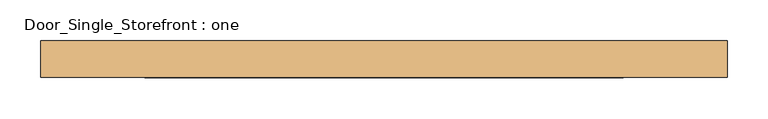
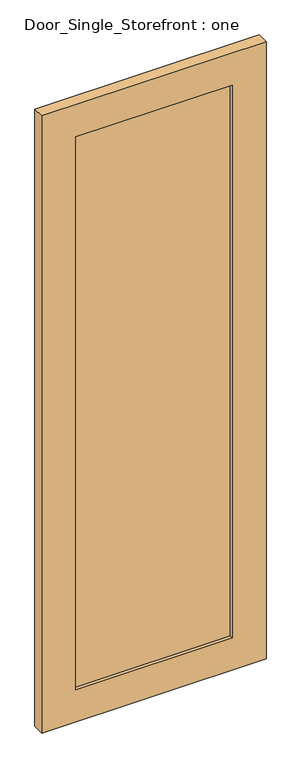
"""IFC4 building model written with IfcOpenShell, lengths in millimetres: door geometry, Door_Single_Storefront : one."""

from ifc_helpers import new_model, si_unit, frame, origin, place, context, project, spatial, polyline, outline, extrude, source, transform, mapped, element, save


def door_single_storefront_one_08b7d5e3(model_context):
    return source(origin(), model_context, "Body", "SweptSolid", [
        extrude(outline(polyline([(292.1, 6.35), (292.1, -12.7), (-292.1, -12.7), (-292.1, 6.35), (292.1, 6.35)])), frame((0.0, 0.0, 127.0), z_axis=(0.0, 0.0, 1.0), x_axis=(1.0, 0.0, 0.0)), (0.0, 0.0, 1.0), 2184.4),
        extrude(outline(polyline([(2438.4, -419.1), (0.0, -419.1), (0.0, 419.1), (2438.4, 419.1), (2438.4, -419.1)]), holes=[polyline([(127.0, 292.1), (127.0, -292.1), (2311.4, -292.1), (2311.4, 292.1), (127.0, 292.1)])]), frame((0.0, -25.4, 0.0), z_axis=(0.0, 1.0, 0.0), x_axis=(0.0, 0.0, 1.0)), (0.0, 0.0, 1.0), 44.45),
    ])


if __name__ == "__main__":
    model = new_model("IFC4")
    model_context = context("Model", 3, world=origin())
    ifc_project = project(units=[si_unit("LENGTHUNIT", "METRE", prefix="MILLI")], contexts=[model_context])
    site = spatial("IfcSite", under=ifc_project)
    building = spatial("IfcBuilding", under=site)
    placement = place(None, origin())
    door_single_storefront_one_shape = door_single_storefront_one_08b7d5e3(model_context)
    element("IfcDoor", 1, ObjectType="Door_Single_Storefront : one", at=placement, inside=building, context=model_context, shape_type="MappedRepresentation", body=[
        mapped(door_single_storefront_one_shape, transform((0.0, 0.0, 0.0), x_axis=(1.0, 0.0, 0.0), y_axis=(0.0, 1.0, 0.0), z_axis=(0.0, 0.0, 1.0))),
    ])
    save(model, "model.ifc")

# Revit data of these elements
# Type "Door_Single_Storefront : one"
#   Type Mark = "27"
#   Analytic Construction = "<None>"
#   Stile_Width = 0' - 5"
#   Door_Thickness = 0' - 1 3/4"
#   Door_Offset = 0' - 1"
#   Glass_Material = SAFETY GLAZING
#   Frame_Material = INTERIOR GRADE ALUMINUM STOREFRONT W/ SAFETY GLAZING
#   Function = (empty or 0)
# Element 1 (IfcDoor, "Door_Single_Storefront : one")
#   Materials on its faces: "INTERIOR GRADE ALUMINUM STOREFRONT W/ SAFETY GLAZING", "SAFETY GLAZING"
# Materials
#   "SAFETY GLAZING": class "Glass", colour RGB 142 168 196, transparency 0.75, Description = "Soda Lime Glass", Cost = 0
#   "INTERIOR GRADE ALUMINUM STOREFRONT W/ SAFETY GLAZING": class "Metal", colour RGB 226 226 226, transparency 0, Description = "Aluminum 6061", Cost = 0
